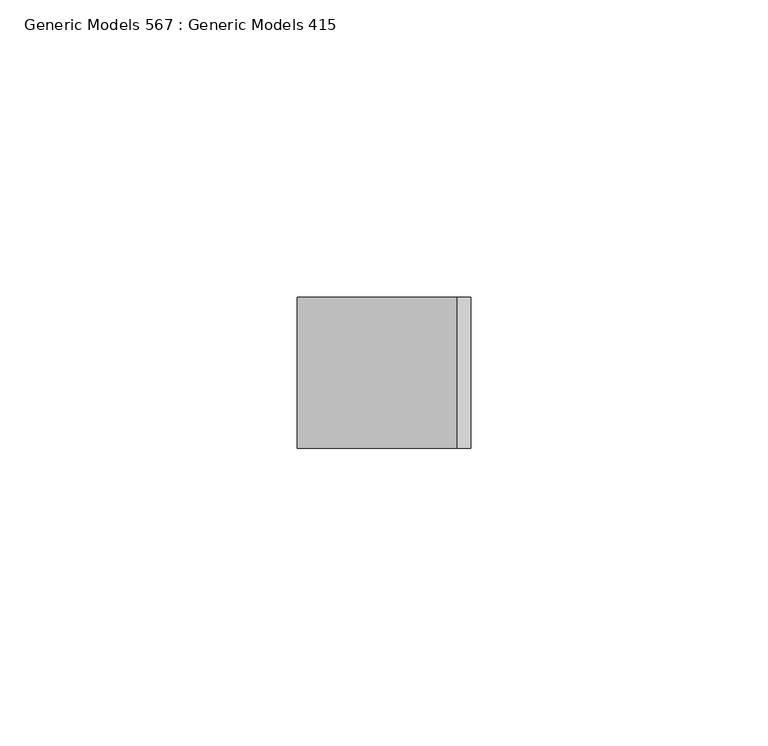
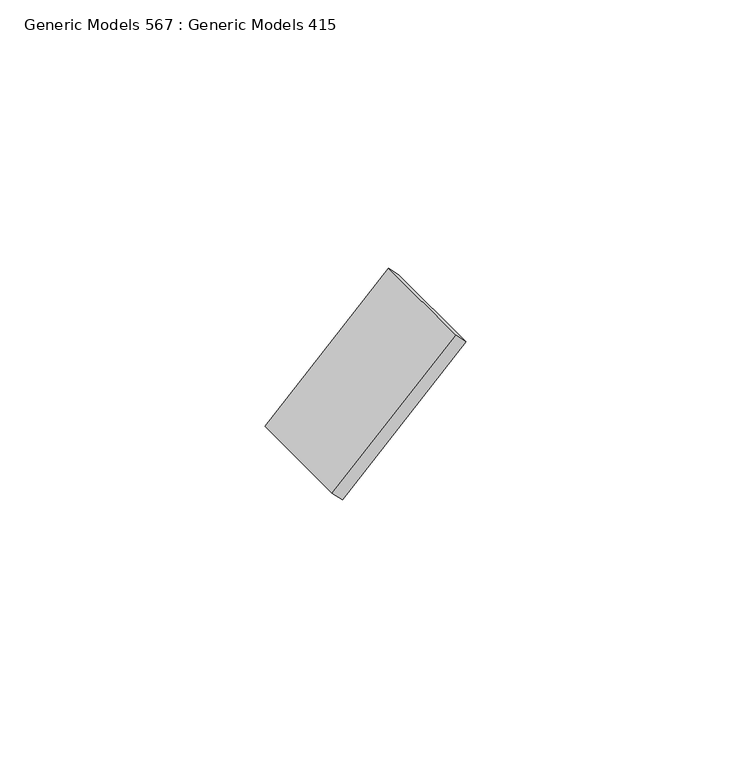
"""IFC4 building model written with IfcOpenShell, lengths in millimetres: proxy geometry, Generic Models 567 : Generic Models 415."""

from ifc_helpers import new_model, si_unit, frame, origin, place, context, project, spatial, polyline, outline, extrude, source, transform, mapped, element, save


def generic_models_567_generic_models_415_70075df2(model_context):
    return source(origin(), model_context, "Body", "SweptSolid", [
        extrude(outline(polyline([(0.0, -3.175), (0.0, 0.0), (25.4, 0.0), (25.4, -3.175), (0.0, -3.175)])), frame((7848.0411784, 4501.3863946, 124178.3849742), z_axis=(0.7071067811867181, 0.0, 0.707106781186377), x_axis=(0.0, -1.0, 0.0)), (0.0, 0.0, 1.0), 38.1),
    ])


if __name__ == "__main__":
    model = new_model("IFC4")
    model_context = context("Model", 3, world=origin())
    ifc_project = project(units=[si_unit("LENGTHUNIT", "METRE", prefix="MILLI")], contexts=[model_context])
    site = spatial("IfcSite", under=ifc_project)
    building = spatial("IfcBuilding", under=site)
    placement = place(None, origin())
    generic_models_567_generic_models_415_shape = generic_models_567_generic_models_415_70075df2(model_context)
    element("IfcBuildingElementProxy", 1, Name="Generic Models 567 : Generic Models 415", ObjectType="Generic Models 567 : Generic Models 415", at=placement, inside=building, context=model_context, shape_type="MappedRepresentation", body=[
        mapped(generic_models_567_generic_models_415_shape, transform((0.0, 0.0, 0.0), x_axis=(1.0, 0.0, 0.0), y_axis=(0.0, 1.0, 0.0), z_axis=(0.0, 0.0, 1.0))),
    ])
    save(model, "model.ifc")

# Revit data of these elements
# Element 1 (IfcBuildingElementProxy, "Generic Models 567 : Generic Models 415")
#   Materials on its faces: "_WELDED STEEL TABS FOR LOUVER ATTACHMENT"
# Materials
#   "_WELDED STEEL TABS FOR LOUVER ATTACHMENT": class "Metal", colour RGB 199 199 199, transparency 0, Description = "Structural steel 50ksi", Cost = 0
